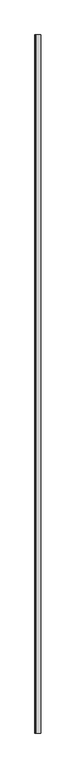
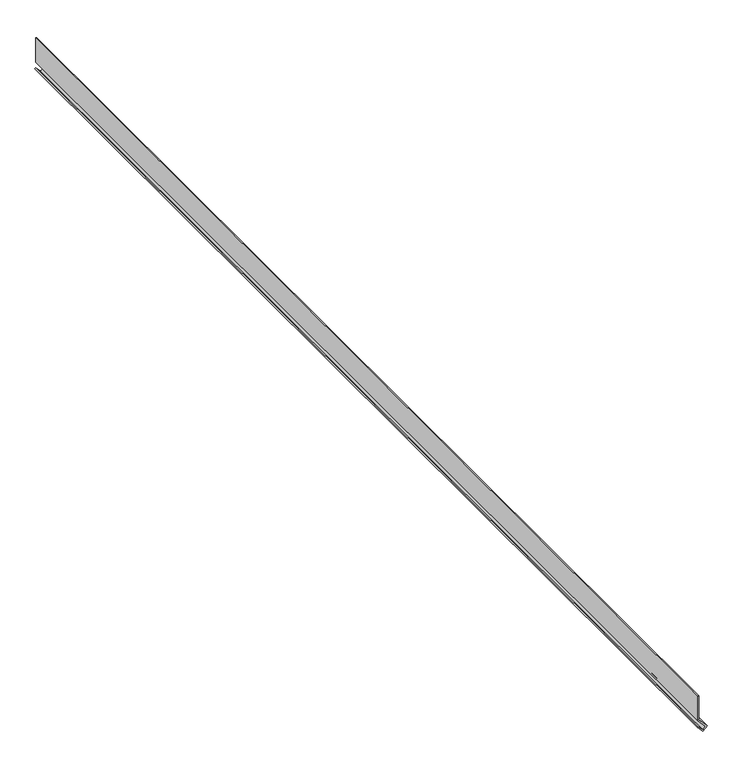
"""IFC4 building model written with IfcOpenShell, lengths in millimetres: proxy geometry, Flashing11:Flashing021:293275 : Flashing11:Flashing021:293275."""

from ifc_helpers import new_model, si_unit, frame, origin, place, context, project, spatial, polyline, outline, extrude, source, transform, mapped, element, save


def generic_models_7d059f76(model_context):
    return source(origin(), model_context, "Body", "SweptSolid", [
        extrude(outline(polyline([(43053.53125, 21428.7571549), (43008.8710938, 21428.7571549), (42993.6445313, 21442.2239517), (42989.0546875, 21437.4407486), (42998.2304688, 21429.1438736), (42996.8890886, 21427.6603982), (42986.1852076, 21437.3390033), (42993.5310498, 21444.9943087), (43009.6286352, 21430.7571549), (43053.53125, 21430.7571549), (43053.53125, 21428.7571549)])), frame((0.0, 8260.4761084, 0.0), z_axis=(0.0, 1.0, 0.0), x_axis=(0.0, 0.0, 1.0)), (0.0, 0.0, 1.0), 2000.0),
    ])


if __name__ == "__main__":
    model = new_model("IFC4")
    model_context = context("Model", 3, world=origin())
    ifc_project = project(units=[si_unit("LENGTHUNIT", "METRE", prefix="MILLI")], contexts=[model_context])
    site = spatial("IfcSite", under=ifc_project)
    building = spatial("IfcBuilding", under=site)
    placement = place(None, origin())
    generic_models_shape = generic_models_7d059f76(model_context)
    element("IfcBuildingElementProxy", 1, Name="Flashing11:Flashing021:293275 : Flashing11:Flashing021:293275", ObjectType="Flashing11:Flashing021:293275 : Flashing11:Flashing021:293275", at=placement, inside=building, context=model_context, shape_type="MappedRepresentation", body=[
        mapped(generic_models_shape, transform((0.0, 0.0, 0.0), x_axis=(1.0, 0.0, 0.0), y_axis=(0.0, 1.0, 0.0), z_axis=(0.0, 0.0, 1.0))),
    ])
    save(model, "model.ifc")

# Revit data of these elements
# Type "Flashing11:Flashing021:293275 : Flashing11:Flashing021:293275"
#   NameOverride = "Flashing11:Flashing021:293275"
#   ObjectTypeOverride = "Flashing11:Flashing021"
#   Reference = "Flashing021"
#   Category = "Generic Models"
#   Tag = "293275"
# Element 1 (IfcBuildingElementProxy, "Flashing11:Flashing021:293275 : Flashing11:Flashing021:293275")
#   Materials on its faces: "16GA. COPPER BRAKE METAL FLASHING"
# Materials
#   "16GA. COPPER BRAKE METAL FLASHING": class "Unassigned", colour RGB 128 128 128, transparency 0, Cost = 0
